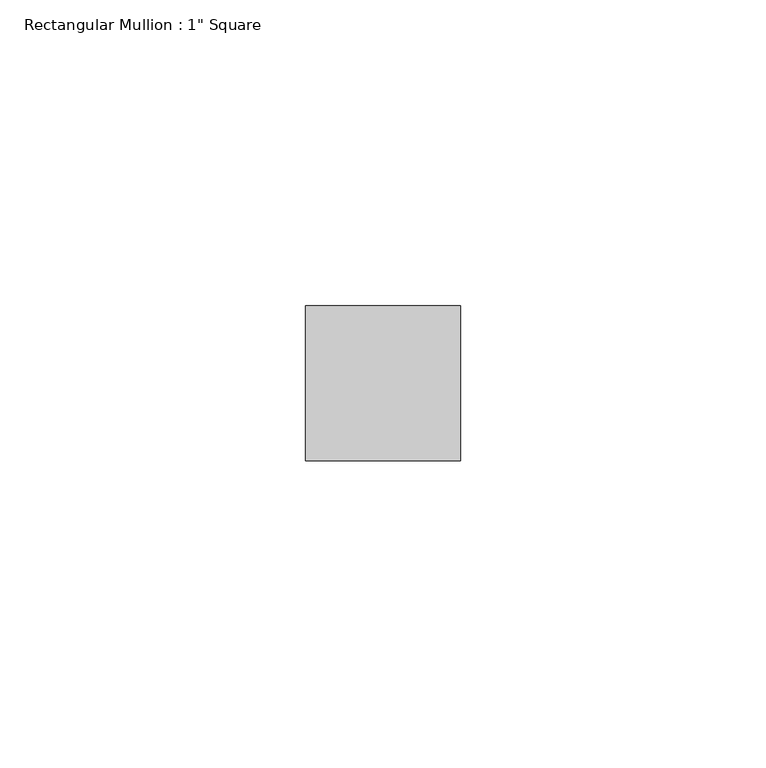
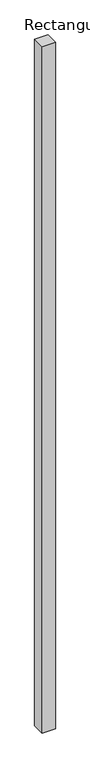
"""IFC4 building model written with IfcOpenShell, lengths in millimetres: member geometry."""

import ifcopenshell
import ifcopenshell.guid

model = None  # the IFC model being written
_history = None  # IfcOwnerHistory: only IFC2X3 demands one
_inside = {}  # id of a spatial element -> (the spatial element, [elements in it])
_under = {}  # id of a project, library or spatial element -> (it, [spatial elements below it])
_declared = {}  # id of a project -> (the project, [libraries it declares])
_typed = {}  # id of a type object -> (the type object, [elements of that type])
_made_of = {}  # id of a material, layer set ... -> (it, [elements and type objects made of it])


def new_model(schema):
    """Start an empty IFC model of exactly this schema.

    Asked for "IFC4X3", IfcOpenShell would pick the latest addendum, in which some entities
    have other attributes; the version numbers below select the first issue.
    IFC2X3 requires an IfcOwnerHistory on every rooted entity: one is made here for all.
    """
    global model, _history
    if schema == "IFC4X3":
        model = ifcopenshell.file(schema_version=(4, 3, 0, 0))
    else:
        model = ifcopenshell.file(schema=schema)
    _inside.clear()
    _under.clear()
    _declared.clear()
    _typed.clear()
    _made_of.clear()
    _history = None
    if model.schema == "IFC2X3":
        org = make("IfcOrganization", Name="unknown")
        user = make(
            "IfcPersonAndOrganization",
            ThePerson=make("IfcPerson", FamilyName="unknown"),
            TheOrganization=org,
        )
        app = make(
            "IfcApplication",
            ApplicationDeveloper=org,
            Version="unknown",
            ApplicationFullName="unknown",
            ApplicationIdentifier="unknown",
        )
        _history = make(
            "IfcOwnerHistory",
            OwningUser=user,
            OwningApplication=app,
            ChangeAction="ADDED",
            CreationDate=0,
        )
    return model


def make(cls, **values):
    """One entity of the class cls with the attributes given. An attribute that is None is left unset."""
    return model.create_entity(
        cls, **{name: value for name, value in values.items() if value is not None}
    )


def rooted(cls, **values):
    """An entity with a GlobalId (a new one), such as an element, a storey or a relation."""
    return make(cls, GlobalId=ifcopenshell.guid.new(), OwnerHistory=_history, **values)


def si_unit(unit_type, name, prefix=None):
    """IfcSIUnit, for example si_unit("LENGTHUNIT", "METRE", prefix="MILLI")."""
    return make("IfcSIUnit", UnitType=unit_type, Prefix=prefix, Name=name)


def assignment(units):
    """IfcUnitAssignment: the units of a project."""
    return None if units is None else make("IfcUnitAssignment", Units=units)


def point(xyz):
    """IfcCartesianPoint."""
    return None if xyz is None else make("IfcCartesianPoint", Coordinates=xyz)


def direction(xyz):
    """IfcDirection."""
    return None if xyz is None else make("IfcDirection", DirectionRatios=xyz)


def frame(location, z_axis=None, x_axis=None):
    """IfcAxis2Placement3D, a coordinate frame: its origin and axes. An axis left out is left unset."""
    return make(
        "IfcAxis2Placement3D",
        Location=point(location),
        Axis=direction(z_axis),
        RefDirection=direction(x_axis),
    )


def origin():
    """The frame at (0, 0, 0) with its axes left unset."""
    return frame((0.0, 0.0, 0.0))


def place(relative_to, where):
    """IfcLocalPlacement: puts the frame where relative to a parent placement (None: the world)."""
    return make(
        "IfcLocalPlacement", PlacementRelTo=relative_to, RelativePlacement=where
    )


def context(
    kind, dimensions, precision=None, world=None, true_north=None, identifier=None
):
    """IfcGeometricRepresentationContext, for example the 3D "Model" context."""
    return make(
        "IfcGeometricRepresentationContext",
        ContextIdentifier=identifier,
        ContextType=kind,
        CoordinateSpaceDimension=dimensions,
        Precision=precision,
        WorldCoordinateSystem=world,
        TrueNorth=true_north,
    )


def project(units=None, contexts=None):
    """IfcProject with its units and contexts."""
    return rooted(
        "IfcProject",
        Name="project",
        RepresentationContexts=contexts,
        UnitsInContext=assignment(units),
    )


def spatial(cls, under=None, at=None, **own):
    """A site, building, storey or space (cls), placed at a placement, below another one or the project."""
    s = rooted(cls, ObjectPlacement=at, **own)
    if under is not None:
        _under.setdefault(under.id(), (under, []))[1].append(s)
    return s


def polyline(points):
    """IfcPolyline through the points."""
    return make("IfcPolyline", Points=[point(p) for p in points])


def outline(outer, holes=None, kind="AREA"):
    """IfcArbitraryClosedProfileDef: a profile drawn as a closed curve; with holes, ...WithVoids."""
    if holes is None:
        return make("IfcArbitraryClosedProfileDef", ProfileType=kind, OuterCurve=outer)
    return make(
        "IfcArbitraryProfileDefWithVoids",
        ProfileType=kind,
        OuterCurve=outer,
        InnerCurves=holes,
    )


def extrude(swept, where, along, depth):
    """IfcExtrudedAreaSolid: the profile swept, set in the frame where, extruded along a direction by depth."""
    return make(
        "IfcExtrudedAreaSolid",
        SweptArea=swept,
        Position=where,
        ExtrudedDirection=direction(along),
        Depth=depth,
    )


def shape(context_of_items, identifier, shape_type, items):
    """IfcShapeRepresentation: the items that make up one representation, for example the "Body"."""
    return make(
        "IfcShapeRepresentation",
        ContextOfItems=context_of_items,
        RepresentationIdentifier=identifier,
        RepresentationType=shape_type,
        Items=items,
    )


def source(mapping_origin, context_of_items, identifier, shape_type, items):
    """IfcRepresentationMap: a shape defined once, which mapped items show again and again."""
    return make(
        "IfcRepresentationMap",
        MappingOrigin=mapping_origin,
        MappedRepresentation=shape(context_of_items, identifier, shape_type, items),
    )


def transform(
    local_origin,
    x_axis=None,
    y_axis=None,
    z_axis=None,
    scale=None,
    scale2=None,
    scale3=None,
    uniform=True,
):
    """IfcCartesianTransformationOperator3D, or its non-uniform kind. x_axis, y_axis, z_axis: its Axis1, 2, 3."""
    if uniform:
        return make(
            "IfcCartesianTransformationOperator3D",
            Axis1=direction(x_axis),
            Axis2=direction(y_axis),
            LocalOrigin=point(local_origin),
            Scale=scale,
            Axis3=direction(z_axis),
        )
    return make(
        "IfcCartesianTransformationOperator3DnonUniform",
        Axis1=direction(x_axis),
        Axis2=direction(y_axis),
        LocalOrigin=point(local_origin),
        Scale=scale,
        Axis3=direction(z_axis),
        Scale2=scale2,
        Scale3=scale3,
    )


def mapped(mapping_source, mapping_target):
    """IfcMappedItem: shows the shape of a source again, moved by a transform."""
    return make(
        "IfcMappedItem", MappingSource=mapping_source, MappingTarget=mapping_target
    )


def made_of(thing, what):
    """Note that an element or type object is made of a material, layer set ...; save() writes the relation."""
    if what is not None:
        _made_of.setdefault(what.id(), (what, []))[1].append(thing)
    return thing


def element(
    cls,
    number,
    at=None,
    inside=None,
    cuts=None,
    type_object=None,
    material=None,
    context=None,
    identifier="Body",
    shape_type=None,
    held_by="IfcProductDefinitionShape",
    body=None,
    shapes=None,
    **own,
):
    """One element of the class cls, such as IfcWall. Its Tag is "e" and its number.

    at: its placement. inside: the storey or other place that contains it. cuts: it is an
    opening in that element (IfcRelVoidsElement). A single representation is given by context,
    identifier, shape_type and body (its items); several are given by shapes. held_by: the class
    of the entity that holds the representations. save() writes the other relations.
    """
    e = rooted(cls, Tag="e%d" % number, ObjectPlacement=at, **own)
    if body is not None:
        shapes = [shape(context, identifier, shape_type, body)]
    if shapes is not None:
        e.Representation = make(held_by, Representations=shapes)
    if inside is not None:
        _inside.setdefault(inside.id(), (inside, []))[1].append(e)
    if cuts is not None:
        rooted(
            "IfcRelVoidsElement", RelatingBuildingElement=cuts, RelatedOpeningElement=e
        )
    if type_object is not None:
        _typed.setdefault(type_object.id(), (type_object, []))[1].append(e)
    return made_of(e, material)


def aggregate(whole, parts):
    """IfcRelAggregates: a whole, such as a stair, and the parts it consists of."""
    return rooted("IfcRelAggregates", RelatingObject=whole, RelatedObjects=parts)


def save(model, path):
    """Write the relations noted so far, then the file.

    IfcRelAggregates (storeys below a building ...), IfcRelContainedInSpatialStructure (elements
    in a storey), IfcRelDefinesByType, IfcRelAssociatesMaterial and IfcRelDeclares: one each for
    every whole, place, type object, material and project.
    """
    for whole, parts in _under.values():
        aggregate(whole, parts)
    for where, things in _inside.values():
        rooted(
            "IfcRelContainedInSpatialStructure",
            RelatedElements=things,
            RelatingStructure=where,
        )
    for kind, things in _typed.values():
        rooted("IfcRelDefinesByType", RelatedObjects=things, RelatingType=kind)
    for what, things in _made_of.values():
        rooted("IfcRelAssociatesMaterial", RelatedObjects=things, RelatingMaterial=what)
    for by, libraries in _declared.values():
        rooted("IfcRelDeclares", RelatingContext=by, RelatedDefinitions=libraries)
    model.write(path)


def member_3258827f(model_context):
    return source(origin(), model_context, "Body", "SweptSolid", [
        extrude(outline(polyline([(0.0, 12.7), (0.0, -12.7), (-25.4, -12.7), (-25.4, 12.7), (0.0, 12.7)])), frame((0.0, 0.0, -1406.525), z_axis=(0.0, 0.0, 1.0), x_axis=(1.0, 0.0, 0.0)), (0.0, 0.0, 1.0), 1406.525),
    ])


if __name__ == "__main__":
    model = new_model("IFC4")
    model_context = context("Model", 3, world=origin())
    ifc_project = project(units=[si_unit("LENGTHUNIT", "METRE", prefix="MILLI")], contexts=[model_context])
    site = spatial("IfcSite", under=ifc_project)
    building = spatial("IfcBuilding", under=site)
    placement = place(None, origin())
    member_shape = member_3258827f(model_context)
    element("IfcMember", 1, ObjectType="Rectangular Mullion : 1\" Square", at=placement, inside=building, context=model_context, shape_type="MappedRepresentation", body=[
        mapped(member_shape, transform((0.0, 0.0, 0.0), x_axis=(1.0, 0.0, 0.0), y_axis=(0.0, 1.0, 0.0), z_axis=(0.0, 0.0, 1.0))),
    ])
    save(model, "model.ifc")

# Revit data of these elements
# Type "Rectangular Mullion : 1\" Square"
#   built-in parameter 1007304 = 0.0833333 (stored number, unit not read)
#   built-in parameter 1007301 = 0.0416667 (stored number, unit not read)
#   built-in parameter 1007300 = 0.0416667 (stored number, unit not read)
# Element 1 (IfcMember, "Rectangular Mullion : 1\" Square")
#   Materials on its faces: "Metal - Aluminum"
# Materials
#   "Metal - Aluminum": class "Metal", colour RGB 247 247 247, transparency 0
